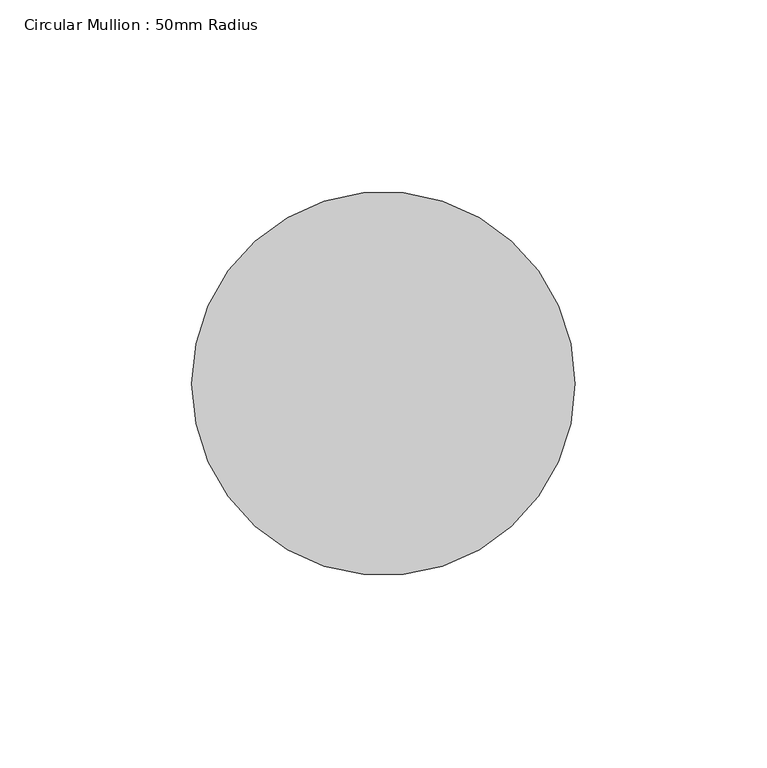
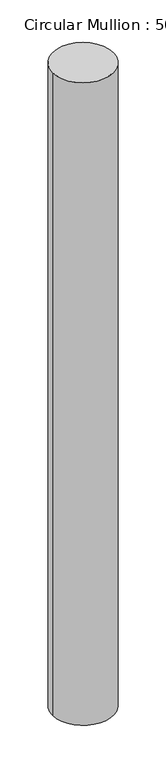
"""IFC4 building model written with IfcOpenShell, lengths in millimetres: member geometry, Circular Mullion : 50mm Radius."""

from ifc_helpers import new_model, si_unit, point, frame, origin, origin_2d, place, context, project, spatial, circle_curve, trimmed, segment, composite_curve, outline, extrude, source, transform, mapped, element, save


def circular_mullion_50mm_radius_d43f5805(model_context):
    return source(origin(), model_context, "Body", "SweptSolid", [
        extrude(outline(composite_curve([segment(trimmed(circle_curve(origin_2d(), 50.0), [point((50.0, 0.0))], [point((-50.0, 0.0))], False, "CARTESIAN"), True, "CONTINUOUS"), segment(trimmed(circle_curve(origin_2d(), 50.0), [point((-50.0, 0.0))], [point((50.0, 0.0))], False, "CARTESIAN"), True, "CONTINUOUS")], self_intersect=False)), frame((0.0, 0.0, -1116.9166426), z_axis=(0.0, 0.0, 1.0), x_axis=(1.0, 0.0, 0.0)), (0.0, 0.0, 1.0), 1116.9166426),
    ])


if __name__ == "__main__":
    model = new_model("IFC4")
    model_context = context("Model", 3, world=origin())
    ifc_project = project(units=[si_unit("LENGTHUNIT", "METRE", prefix="MILLI")], contexts=[model_context])
    site = spatial("IfcSite", under=ifc_project)
    building = spatial("IfcBuilding", under=site)
    placement = place(None, origin())
    circular_mullion_50mm_radius_shape = circular_mullion_50mm_radius_d43f5805(model_context)
    element("IfcMember", 1, ObjectType="Circular Mullion : 50mm Radius", at=placement, inside=building, context=model_context, shape_type="MappedRepresentation", body=[
        mapped(circular_mullion_50mm_radius_shape, transform((0.0, 0.0, 0.0), x_axis=(1.0, 0.0, 0.0), y_axis=(0.0, 1.0, 0.0), z_axis=(0.0, 0.0, 1.0))),
    ])
    save(model, "model.ifc")

# Revit data of these elements
# Type "Circular Mullion : 50mm Radius"
#   built-in parameter 1007350 = 0.164042 (stored number, unit not read)
# Element 1 (IfcMember, "Circular Mullion : 50mm Radius")
#   Materials on its faces: "Aluminium"
# Materials
#   "Aluminium": class "Metal", colour RGB 247 247 247, transparency 0, Description = "Aluminium 6061", Cost = 0
